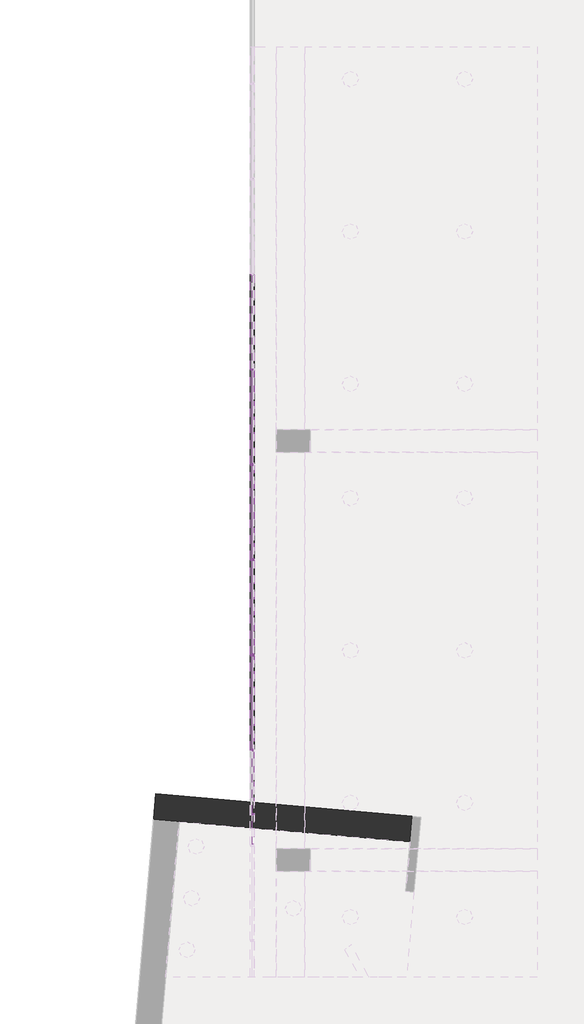
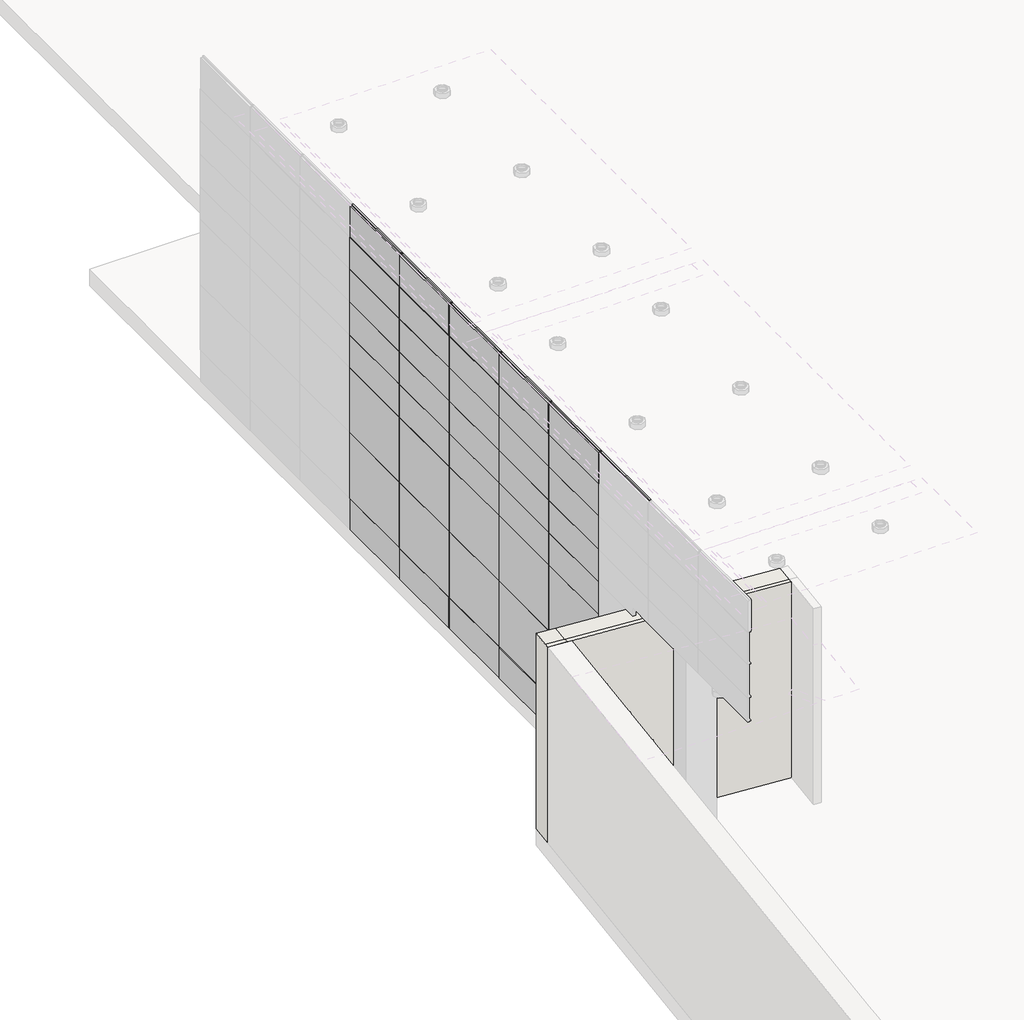
# One storey, part 6 of 30: 90 members, 40 plates, 1 wall.
# Revit data of these elements (continued)
# Space at (-48636.12, -949.776) mm, phase "New Construction", upper level "1ST. FL.", upper offset 3048 mm, lower offset 0 mm (continued)
#   Return Airflow = 0
#   Occupancy Unit = -1
#   Condition Type = 2
#   Construction Type = none
# Space at (-24605.823, -26109.518) mm, phase "New Construction", upper level "1ST. FL.", upper offset 3048 mm, lower offset 0 mm
#   Number = "165"
#   Name = "Space"
#   Actual Lighting Load per area = 0
#   Actual Power Load per area = 0
#   Sensible Heat Gain per person = 0
#   Specified Lighting Load = 11573.5 (stored number, unit not read)
#   Specified Power Load = 15045.5 (stored number, unit not read)
#   Latent Heat Gain per person = 0
#   Total Heat Gain per person = 0
#   Area per Person = 0
#   Number of People = 3.49616 (stored number, unit not read)
#   Lighting Load Units = 0
#   Power Load Units = 0
#   Return Airflow = 0
#   Occupancy Unit = -1
#   Condition Type = 2
#   Construction Type = none
# Space at (-26178.864, -19923.037) mm, phase "New Construction", upper level "1ST. FL.", upper offset 3048 mm, lower offset 0 mm
#   Number = "166"
#   Name = "Space"
#   Actual Lighting Load per area = 0
#   Actual Power Load per area = 0
#   Sensible Heat Gain per person = 0
#   Specified Lighting Load = 6526.22 (stored number, unit not read)
#   Specified Power Load = 8484.08 (stored number, unit not read)
#   Latent Heat Gain per person = 0
#   Total Heat Gain per person = 0
#   Area per Person = 0
#   Number of People = 1.97147 (stored number, unit not read)
#   Lighting Load Units = 0
#   Power Load Units = 0
#   Return Airflow = 0
#   Occupancy Unit = -1
#   Condition Type = 2
#   Construction Type = none
# Space at (-31002.156, -29519.268) mm, phase "New Construction", upper level "1ST. FL.", upper offset 3048 mm, lower offset 0 mm
#   Number = "167"
#   Name = "Space"
#   Actual Lighting Load per area = 0
#   Actual Power Load per area = 0
#   Sensible Heat Gain per person = 0
#   Specified Lighting Load = 1751.97 (stored number, unit not read)
#   Specified Power Load = 2277.57 (stored number, unit not read)
#   Latent Heat Gain per person = 0
#   Total Heat Gain per person = 0
#   Area per Person = 0
#   Number of People = 0.529244 (stored number, unit not read)
#   Lighting Load Units = 0
#   Power Load Units = 0
#   Return Airflow = 0
#   Occupancy Unit = -1
#   Condition Type = 2
#   Construction Type = none
# Space at (-35232.658, -22961.72) mm, phase "New Construction", upper level "1ST. FL.", upper offset 3048 mm, lower offset 0 mm
#   Number = "168"
#   Name = "Space"
#   Actual Lighting Load per area = 0
#   Actual Power Load per area = 0
#   Sensible Heat Gain per person = 0
#   Specified Lighting Load = 14661.4 (stored number, unit not read)
#   Specified Power Load = 19059.8 (stored number, unit not read)
#   Latent Heat Gain per person = 0
#   Total Heat Gain per person = 0
#   Area per Person = 0
#   Number of People = 4.42898 (stored number, unit not read)
#   Lighting Load Units = 0
#   Power Load Units = 0
#   Return Airflow = 0
#   Occupancy Unit = -1
#   Condition Type = 2
#   Construction Type = none
# Space at (-44559.948, -27773.147) mm, phase "New Construction", upper level "1ST. FL.", upper offset 3048 mm, lower offset 0 mm
#   Number = "6"
#   Name = "Space"
#   Actual Lighting Load per area = 0
#   Actual Power Load per area = 0
#   Sensible Heat Gain per person = 0
#   Specified Lighting Load = 153.554 (stored number, unit not read)
#   Specified Power Load = 199.62 (stored number, unit not read)
#   Latent Heat Gain per person = 0
#   Total Heat Gain per person = 0
#   Area per Person = 0
#   Number of People = 0.0463862 (stored number, unit not read)
#   Lighting Load Units = 0
#   Power Load Units = 0
#   Return Airflow = 0
#   Occupancy Unit = -1
#   Condition Type = 2
#   Construction Type = none
# Space at (-44641.303, -28703.045) mm, phase "New Construction", upper level "1ST. FL.", upper offset 3048 mm, lower offset 0 mm
#   Number = "7"
#   Name = "Space"
#   Actual Lighting Load per area = 0
#   Actual Power Load per area = 0
#   Sensible Heat Gain per person = 0
#   Specified Lighting Load = 153.554 (stored number, unit not read)
#   Specified Power Load = 199.62 (stored number, unit not read)
#   Latent Heat Gain per person = 0
#   Total Heat Gain per person = 0
#   Area per Person = 0
#   Number of People = 0.0463862 (stored number, unit not read)
#   Lighting Load Units = 0
#   Power Load Units = 0
#   Return Airflow = 0
#   Occupancy Unit = -1
#   Condition Type = 2
#   Construction Type = none
# Space at (-44722.659, -29632.943) mm, phase "New Construction", upper level "1ST. FL.", upper offset 3048 mm, lower offset 0 mm
#   Number = "8"
#   Name = "Space"
#   Actual Lighting Load per area = 0
#   Actual Power Load per area = 0
#   Sensible Heat Gain per person = 0
#   Specified Lighting Load = 153.554 (stored number, unit not read)
#   Specified Power Load = 199.62 (stored number, unit not read)
#   Latent Heat Gain per person = 0
#   Total Heat Gain per person = 0
#   Area per Person = 0
#   Number of People = 0.0463862 (stored number, unit not read)
#   Lighting Load Units = 0
#   Power Load Units = 0
#   Return Airflow = 0
#   Occupancy Unit = -1
#   Condition Type = 2
#   Construction Type = none
# Space at (4481.556, -17544.26) mm, phase "New Construction", upper level "1ST. FL.", upper offset 3048 mm, lower offset 0 mm
#   Number = "26"
#   Name = "Space"
#   Actual Lighting Load per area = 0
#   Actual Power Load per area = 0
#   Sensible Heat Gain per person = 0
#   Specified Lighting Load = 668.56 (stored number, unit not read)
#   Specified Power Load = 869.128 (stored number, unit not read)
#   Latent Heat Gain per person = 0
#   Total Heat Gain per person = 0
#   Area per Person = 0
#   Number of People = 0.201961 (stored number, unit not read)
#   Lighting Load Units = 0
#   Power Load Units = 0
#   Return Airflow = 0
#   Occupancy Unit = -1
#   Condition Type = 2
#   Construction Type = none
# Space at (13610.668, -16864.797) mm, phase "New Construction", upper level "1ST. FL.", upper offset 3048 mm, lower offset 0 mm
#   Number = "27"
#   Name = "Space"
#   Actual Lighting Load per area = 0
#   Actual Power Load per area = 0
#   Sensible Heat Gain per person = 0
#   Specified Lighting Load = 754.308 (stored number, unit not read)
#   Specified Power Load = 980.601 (stored number, unit not read)
#   Latent Heat Gain per person = 0
#   Total Heat Gain per person = 0
#   Area per Person = 0
#   Number of People = 0.227865 (stored number, unit not read)
#   Lighting Load Units = 0
#   Power Load Units = 0
#   Return Airflow = 0
#   Occupancy Unit = -1
#   Condition Type = 2
#   Construction Type = none
# Space at (16138.502, -11083.135) mm, phase "New Construction", upper level "1ST. FL.", upper offset 3048 mm, lower offset 0 mm
#   Number = "28"
#   Name = "Space"
#   Actual Lighting Load per area = 0
#   Actual Power Load per area = 0
#   Sensible Heat Gain per person = 0
#   Specified Lighting Load = 89.5362 (stored number, unit not read)
#   Specified Power Load = 116.397 (stored number, unit not read)
#   Latent Heat Gain per person = 0
#   Total Heat Gain per person = 0
#   Area per Person = 0
#   Number of People = 0.0270475 (stored number, unit not read)
#   Lighting Load Units = 0
#   Power Load Units = 0
#   Return Airflow = 0
#   Occupancy Unit = -1
#   Condition Type = 2
#   Construction Type = none
# Space at (-40541.142, -26152.586) mm, phase "New Construction", upper level "1ST. FL.", upper offset 3048 mm, lower offset 0 mm
#   Number = "3"
#   Name = "Space"
#   Actual Lighting Load per area = 0
#   Actual Power Load per area = 0
#   Sensible Heat Gain per person = 0
#   Specified Lighting Load = 4.78874 (stored number, unit not read)
#   Specified Power Load = 6.22536 (stored number, unit not read)
#   Latent Heat Gain per person = 0
#   Total Heat Gain per person = 0
#   Area per Person = 0
#   Number of People = 0.0014466 (stored number, unit not read)
#   Lighting Load Units = 0
#   Power Load Units = 0
#   Return Airflow = 0
#   Occupancy Unit = -1
#   Condition Type = 2
#   Construction Type = none
# Space at (-17133.844, -17937.396) mm, phase "New Construction", upper level "1ST. FL.", upper offset 3048 mm, lower offset 0 mm
#   Number = "32"
#   Name = "Space"
#   Actual Lighting Load per area = 0
#   Actual Power Load per area = 0
#   Sensible Heat Gain per person = 0
#   Specified Lighting Load = 933.723 (stored number, unit not read)
#   Specified Power Load = 1213.84 (stored number, unit not read)
#   Latent Heat Gain per person = 0
#   Total Heat Gain per person = 0
#   Area per Person = 0
#   Number of People = 0.282063 (stored number, unit not read)
#   Lighting Load Units = 0
#   Power Load Units = 0
#   Return Airflow = 0
#   Occupancy Unit = -1
#   Condition Type = 2
#   Construction Type = none
# Space at (-14581.144, -19075.025) mm, phase "New Construction", upper level "1ST. FL.", upper offset 3048 mm, lower offset 0 mm
#   Number = "33"
#   Name = "Space"
#   Actual Lighting Load per area = 0
#   Actual Power Load per area = 0
#   Sensible Heat Gain per person = 0
#   Specified Lighting Load = 79.3036 (stored number, unit not read)
#   Specified Power Load = 103.095 (stored number, unit not read)
#   Latent Heat Gain per person = 0
#   Total Heat Gain per person = 0
#   Area per Person = 0
#   Number of People = 0.0239564 (stored number, unit not read)
#   Lighting Load Units = 0
#   Power Load Units = 0
#   Return Airflow = 0
#   Occupancy Unit = -1
#   Condition Type = 2
#   Construction Type = none
# Space at (-36860.119, -18528.984) mm, phase "New Construction", upper level "1ST. FL.", upper offset 3048 mm, lower offset 0 mm
#   Number = "34"
#   Name = "Space"
#   Actual Lighting Load per area = 0
#   Actual Power Load per area = 0
#   Sensible Heat Gain per person = 0
#   Specified Lighting Load = 2950.45 (stored number, unit not read)
#   Specified Power Load = 3835.59 (stored number, unit not read)
#   Latent Heat Gain per person = 0
#   Total Heat Gain per person = 0
#   Area per Person = 0
#   Number of People = 0.891285 (stored number, unit not read)
#   Lighting Load Units = 0
#   Power Load Units = 0
#   Return Airflow = 0
#   Occupancy Unit = -1
#   Condition Type = 2
#   Construction Type = none
# Space at (15225.756, 13850.14) mm, phase "New Construction", upper level "1ST. FL.", upper offset 3048 mm, lower offset 0 mm
#   Number = "35"
#   Name = "Space"
#   Actual Lighting Load per area = 0
#   Actual Power Load per area = 0
#   Sensible Heat Gain per person = 0
#   Specified Lighting Load = 62.8642 (stored number, unit not read)
#   Specified Power Load = 81.7235 (stored number, unit not read)
#   Latent Heat Gain per person = 0
#   Total Heat Gain per person = 0
#   Area per Person = 0
#   Number of People = 0.0189903 (stored number, unit not read)
#   Lighting Load Units = 0
#   Power Load Units = 0
#   Return Airflow = 0
#   Occupancy Unit = -1
#   Condition Type = 2
#   Construction Type = none
# Space at (-44280.616, -26218.59) mm, phase "New Construction", upper level "1ST. FL.", upper offset 3048 mm, lower offset 0 mm
#   Number = "4"
#   Name = "Space"
#   Actual Lighting Load per area = 0
#   Actual Power Load per area = 0
#   Sensible Heat Gain per person = 0
#   Specified Lighting Load = 35.218 (stored number, unit not read)
#   Specified Power Load = 45.7834 (stored number, unit not read)
#   Latent Heat Gain per person = 0
#   Total Heat Gain per person = 0
#   Area per Person = 0
#   Number of People = 0.0106388 (stored number, unit not read)
#   Lighting Load Units = 0
#   Power Load Units = 0
#   Return Airflow = 0
#   Occupancy Unit = -1
#   Condition Type = 2
#   Construction Type = none
# Space at (-44388.044, 13850.14) mm, phase "New Construction", upper level "1ST. FL.", upper offset 3048 mm, lower offset 0 mm
#   Number = "38"
#   Name = "Space"
#   Actual Lighting Load per area = 0
#   Actual Power Load per area = 0
#   Sensible Heat Gain per person = 0
#   Specified Lighting Load = 62.8642 (stored number, unit not read)
#   Specified Power Load = 81.7235 (stored number, unit not read)
#   Latent Heat Gain per person = 0
#   Total Heat Gain per person = 0
#   Area per Person = 0
#   Number of People = 0.0189903 (stored number, unit not read)
#   Lighting Load Units = 0
#   Power Load Units = 0
#   Return Airflow = 0
#   Occupancy Unit = -1
#   Condition Type = 2
#   Construction Type = none
# Space at (-49662.767, -15921.188) mm, phase "New Construction", upper level "1ST. FL.", upper offset 3048 mm, lower offset 0 mm
#   Number = "1"
#   Name = "Space"
#   Actual Lighting Load per area = 0
#   Actual Power Load per area = 0
#   Sensible Heat Gain per person = 0
#   Specified Lighting Load = 10.6063 (stored number, unit not read)
#   Specified Power Load = 13.7882 (stored number, unit not read)
#   Latent Heat Gain per person = 0
#   Total Heat Gain per person = 0
#   Area per Person = 0
#   Number of People = 0.003204 (stored number, unit not read)
#   Lighting Load Units = 0
#   Power Load Units = 0
#   Return Airflow = 0
#   Occupancy Unit = -1
#   Condition Type = 2
#   Construction Type = none
# Space at (-14581.144, 13850.14) mm, phase "New Construction", upper level "1ST. FL.", upper offset 3048 mm, lower offset 0 mm
#   Number = "39"
#   Name = "Space"
#   Actual Lighting Load per area = 0
#   Actual Power Load per area = 0
#   Sensible Heat Gain per person = 0
#   Specified Lighting Load = 134.399 (stored number, unit not read)
#   Specified Power Load = 174.719 (stored number, unit not read)
#   Latent Heat Gain per person = 0
#   Total Heat Gain per person = 0
#   Area per Person = 0
#   Number of People = 0.0405999 (stored number, unit not read)
#   Lighting Load Units = 0
#   Power Load Units = 0
#   Return Airflow = 0
#   Occupancy Unit = -1
#   Condition Type = 2
#   Construction Type = none
# Space at (-27319.244, 18968.24) mm, phase "New Construction", upper level "1ST. FL.", upper offset 3048 mm, lower offset 0 mm
#   Number = "42"
#   Name = "Space"
#   Actual Lighting Load per area = 0
#   Actual Power Load per area = 0
#   Sensible Heat Gain per person = 0
#   Specified Lighting Load = 63.238 (stored number, unit not read)
#   Specified Power Load = 82.2094 (stored number, unit not read)
#   Latent Heat Gain per person = 0
#   Total Heat Gain per person = 0
#   Area per Person = 0
#   Number of People = 0.0191032 (stored number, unit not read)
#   Lighting Load Units = 0
#   Power Load Units = 0
#   Return Airflow = 0
#   Occupancy Unit = -1
#   Condition Type = 2
#   Construction Type = none
# Space at (-26039.719, 18968.24) mm, phase "New Construction", upper level "1ST. FL.", upper offset 3048 mm, lower offset 0 mm
#   Number = "43"
#   Name = "Space"
#   Actual Lighting Load per area = 0
#   Actual Power Load per area = 0
#   Sensible Heat Gain per person = 0
#   Specified Lighting Load = 552.454 (stored number, unit not read)
#   Specified Power Load = 718.19 (stored number, unit not read)
#   Latent Heat Gain per person = 0
#   Total Heat Gain per person = 0
#   Area per Person = 0
#   Number of People = 0.166888 (stored number, unit not read)
#   Lighting Load Units = 0
#   Power Load Units = 0
#   Return Airflow = 0
#   Occupancy Unit = -1
#   Condition Type = 2
#   Construction Type = none
# Space at (15806.781, -12603.96) mm, phase "New Construction", upper level "1ST. FL.", upper offset 3048 mm, lower offset 0 mm
#   Number = "60"
#   Name = "Space"
#   Actual Lighting Load per area = 0
#   Actual Power Load per area = 0
#   Sensible Heat Gain per person = 0
#   Specified Lighting Load = 3.50388 (stored number, unit not read)
#   Specified Power Load = 4.55504 (stored number, unit not read)
#   Latent Heat Gain per person = 0
#   Total Heat Gain per person = 0
#   Area per Person = 0
#   Number of People = 0.00105847 (stored number, unit not read)
#   Lighting Load Units = 0
#   Power Load Units = 0
#   Return Airflow = 0
#   Occupancy Unit = -1
#   Condition Type = 2
#   Construction Type = none
# Space at (-44850.987, -31099.746) mm, phase "New Construction", upper level "1ST. FL.", upper offset 3048 mm, lower offset 0 mm
#   Number = "9"
#   Name = "Space"
#   Actual Lighting Load per area = 0
#   Actual Power Load per area = 0
#   Sensible Heat Gain per person = 0
#   Specified Lighting Load = 352.476 (stored number, unit not read)
#   Specified Power Load = 458.219 (stored number, unit not read)
#   Latent Heat Gain per person = 0
#   Total Heat Gain per person = 0
#   Area per Person = 0
#   Number of People = 0.106477 (stored number, unit not read)
#   Lighting Load Units = 0
#   Power Load Units = 0
#   Return Airflow = 0
#   Occupancy Unit = -1
#   Condition Type = 2
#   Construction Type = none
# Space at (15806.781, -5898.36) mm, phase "New Construction", upper level "1ST. FL.", upper offset 3048 mm, lower offset 0 mm
#   Number = "61"
#   Name = "Space"
#   Actual Lighting Load per area = 0
#   Actual Power Load per area = 0
#   Sensible Heat Gain per person = 0
#   Specified Lighting Load = 3.50388 (stored number, unit not read)
#   Specified Power Load = 4.55504 (stored number, unit not read)
#   Latent Heat Gain per person = 0
#   Total Heat Gain per person = 0
#   Area per Person = 0
#   Number of People = 0.00105847 (stored number, unit not read)
#   Lighting Load Units = 0
#   Power Load Units = 0
#   Return Airflow = 0
#   Occupancy Unit = -1
#   Condition Type = 2
#   Construction Type = none
# Space at (-41141.59, -31068.115) mm, phase "New Construction", upper level "1ST. FL.", upper offset 3048 mm, lower offset 0 mm
#   Number = "2"
#   Name = "Space"
#   Actual Lighting Load per area = 0
#   Actual Power Load per area = 0
#   Sensible Heat Gain per person = 0
#   Specified Lighting Load = 101.303 (stored number, unit not read)
#   Specified Power Load = 131.694 (stored number, unit not read)
#   Latent Heat Gain per person = 0
#   Total Heat Gain per person = 0
#   Area per Person = 0
#   Number of People = 0.030602 (stored number, unit not read)
#   Lighting Load Units = 0
#   Power Load Units = 0
#   Return Airflow = 0
#   Occupancy Unit = -1
#   Condition Type = 2
#   Construction Type = none
# Space at (-46265.71, -27605.083) mm, phase "New Construction", upper level "1ST. FL.", upper offset 3048 mm, lower offset 0 mm
#   Number = "10"
#   Name = "Space"
#   Actual Lighting Load per area = 0
#   Actual Power Load per area = 0
#   Sensible Heat Gain per person = 0
#   Specified Lighting Load = 198.964 (stored number, unit not read)
#   Specified Power Load = 258.653 (stored number, unit not read)
#   Latent Heat Gain per person = 0
#   Total Heat Gain per person = 0
#   Area per Person = 0
#   Number of People = 0.0601039 (stored number, unit not read)
#   Lighting Load Units = 0
#   Power Load Units = 0
#   Return Airflow = 0
#   Occupancy Unit = -1
#   Condition Type = 2
#   Construction Type = none
# Space at (-47287.648, -27585.498) mm, phase "New Construction", upper level "1ST. FL.", upper offset 3048 mm, lower offset 0 mm
#   Number = "11"
#   Name = "Space"
#   Actual Lighting Load per area = 0
#   Actual Power Load per area = 0
#   Sensible Heat Gain per person = 0
#   Specified Lighting Load = 153.554 (stored number, unit not read)
#   Specified Power Load = 199.62 (stored number, unit not read)
#   Latent Heat Gain per person = 0
#   Total Heat Gain per person = 0
#   Area per Person = 0
#   Number of People = 0.0463862 (stored number, unit not read)
#   Lighting Load Units = 0
#   Power Load Units = 0
#   Return Airflow = 0
#   Occupancy Unit = -1
#   Condition Type = 2
#   Construction Type = none
# Space at (-50077.342, -27341.431) mm, phase "New Construction", upper level "1ST. FL.", upper offset 3048 mm, lower offset 0 mm
#   Number = "14"
#   Name = "Space"
#   Actual Lighting Load per area = 0
#   Actual Power Load per area = 0
#   Sensible Heat Gain per person = 0
#   Specified Lighting Load = 153.554 (stored number, unit not read)
#   Specified Power Load = 199.62 (stored number, unit not read)
#   Latent Heat Gain per person = 0
#   Total Heat Gain per person = 0
#   Area per Person = 0
#   Number of People = 0.0463862 (stored number, unit not read)
#   Lighting Load Units = 0
#   Power Load Units = 0
#   Return Airflow = 0
#   Occupancy Unit = -1
#   Condition Type = 2
#   Construction Type = none
# Space at (29814.881, 10827.54) mm, phase "New Construction", upper level "1ST. FL.", upper offset 3048 mm, lower offset 0 mm
#   Number = "86"
#   Name = "Space"
#   Actual Lighting Load per area = 0
#   Actual Power Load per area = 0
#   Sensible Heat Gain per person = 0
#   Specified Lighting Load = 153.554 (stored number, unit not read)
#   Specified Power Load = 199.62 (stored number, unit not read)
#   Latent Heat Gain per person = 0
#   Total Heat Gain per person = 0
#   Area per Person = 0
#   Number of People = 0.0463862 (stored number, unit not read)
#   Lighting Load Units = 0
#   Power Load Units = 0
#   Return Airflow = 0
#   Occupancy Unit = -1
#   Condition Type = 2
#   Construction Type = none
# Space at (-51007.239, -27260.076) mm, phase "New Construction", upper level "1ST. FL.", upper offset 3048 mm, lower offset 0 mm
#   Number = "15"
#   Name = "Space"
#   Actual Lighting Load per area = 0
#   Actual Power Load per area = 0
#   Sensible Heat Gain per person = 0
#   Specified Lighting Load = 153.554 (stored number, unit not read)
#   Specified Power Load = 199.62 (stored number, unit not read)
#   Latent Heat Gain per person = 0
#   Total Heat Gain per person = 0
#   Area per Person = 0
#   Number of People = 0.0463862 (stored number, unit not read)
#   Lighting Load Units = 0
#   Power Load Units = 0
#   Return Airflow = 0
#   Occupancy Unit = -1
#   Condition Type = 2
#   Construction Type = none
# Space at (-47010.699, -30758.61) mm, phase "New Construction", upper level "1ST. FL.", upper offset 3048 mm, lower offset 0 mm
#   Number = "17"
#   Name = "Space"
#   Actual Lighting Load per area = 0
#   Actual Power Load per area = 0
#   Sensible Heat Gain per person = 0
#   Specified Lighting Load = 352.476 (stored number, unit not read)
#   Specified Power Load = 458.219 (stored number, unit not read)
#   Latent Heat Gain per person = 0
#   Total Heat Gain per person = 0
#   Area per Person = 0
#   Number of People = 0.106477 (stored number, unit not read)
#   Lighting Load Units = 0
#   Power Load Units = 0
#   Return Airflow = 0
#   Occupancy Unit = -1
#   Condition Type = 2
#   Construction Type = none
# Space at (28636.162, 6964.942) mm, phase "New Construction", upper level "1ST. FL.", upper offset 3048 mm, lower offset 0 mm
#   Number = "101"
#   Name = "Space"
#   Actual Lighting Load per area = 0
#   Actual Power Load per area = 0
#   Sensible Heat Gain per person = 0
#   Specified Lighting Load = 2584.91 (stored number, unit not read)
#   Specified Power Load = 3360.39 (stored number, unit not read)
#   Latent Heat Gain per person = 0
#   Total Heat Gain per person = 0
#   Area per Person = 0
#   Number of People = 0.780861 (stored number, unit not read)
#   Lighting Load Units = 0
#   Power Load Units = 0
#   Return Airflow = 0
#   Occupancy Unit = -1
#   Condition Type = 2
#   Construction Type = none
# Space at (-25325.344, 24245.09) mm, phase "New Construction", upper level "1ST. FL.", upper offset 3048 mm, lower offset 0 mm
#   Number = "52"
#   Name = "Space"
#   Actual Lighting Load per area = 0
#   Actual Power Load per area = 0
#   Sensible Heat Gain per person = 0
#   Specified Lighting Load = 1393.93 (stored number, unit not read)
#   Specified Power Load = 1812.1 (stored number, unit not read)
#   Latent Heat Gain per person = 0
#   Total Heat Gain per person = 0
#   Area per Person = 0
#   Number of People = 0.421083 (stored number, unit not read)
#   Lighting Load Units = 0
#   Power Load Units = 0
#   Return Airflow = 0
#   Occupancy Unit = -1
#   Condition Type = 2
#   Construction Type = none
# Space at (-48217.546, -27504.142) mm, phase "New Construction", upper level "1ST. FL.", upper offset 3048 mm, lower offset 0 mm
#   Number = "12"
#   Name = "Space"
#   Actual Lighting Load per area = 0
#   Actual Power Load per area = 0
#   Sensible Heat Gain per person = 0
#   Specified Lighting Load = 153.554 (stored number, unit not read)
#   Specified Power Load = 199.62 (stored number, unit not read)
#   Latent Heat Gain per person = 0
#   Total Heat Gain per person = 0
#   Area per Person = 0
#   Number of People = 0.0463862 (stored number, unit not read)
#   Lighting Load Units = 0
#   Power Load Units = 0
#   Return Airflow = 0
#   Occupancy Unit = -1
#   Condition Type = 2
#   Construction Type = none
# Space at (-49147.444, -27422.787) mm, phase "New Construction", upper level "1ST. FL.", upper offset 3048 mm, lower offset 0 mm
#   Number = "13"
#   Name = "Space"
#   Actual Lighting Load per area = 0
#   Actual Power Load per area = 0
#   Sensible Heat Gain per person = 0
#   Specified Lighting Load = 153.554 (stored number, unit not read)
#   Specified Power Load = 199.62 (stored number, unit not read)
#   Latent Heat Gain per person = 0
#   Total Heat Gain per person = 0
#   Area per Person = 0
#   Number of People = 0.0463862 (stored number, unit not read)
#   Lighting Load Units = 0
#   Power Load Units = 0
#   Return Airflow = 0
#   Occupancy Unit = -1
#   Condition Type = 2
#   Construction Type = none
# Space at (-51937.137, -27178.72) mm, phase "New Construction", upper level "1ST. FL.", upper offset 3048 mm, lower offset 0 mm
#   Number = "16"
#   Name = "Space"
#   Actual Lighting Load per area = 0
#   Actual Power Load per area = 0
#   Sensible Heat Gain per person = 0
#   Specified Lighting Load = 153.554 (stored number, unit not read)
#   Specified Power Load = 199.62 (stored number, unit not read)
#   Latent Heat Gain per person = 0
#   Total Heat Gain per person = 0
#   Area per Person = 0
#   Number of People = 0.0463862 (stored number, unit not read)
#   Lighting Load Units = 0
#   Power Load Units = 0
#   Return Airflow = 0
#   Occupancy Unit = -1
#   Condition Type = 2
#   Construction Type = none
# Space at (-48490.944, -30629.106) mm, phase "New Construction", upper level "1ST. FL.", upper offset 3048 mm, lower offset 0 mm
#   Number = "18"
#   Name = "Space"
#   Actual Lighting Load per area = 0
#   Actual Power Load per area = 0
#   Sensible Heat Gain per person = 0
#   Specified Lighting Load = 153.554 (stored number, unit not read)
#   Specified Power Load = 199.62 (stored number, unit not read)
#   Latent Heat Gain per person = 0
#   Total Heat Gain per person = 0
#   Area per Person = 0
#   Number of People = 0.0463862 (stored number, unit not read)
#   Lighting Load Units = 0
#   Power Load Units = 0
#   Return Airflow = 0
#   Occupancy Unit = -1
#   Condition Type = 2
#   Construction Type = none
# Space at (-49420.842, -30547.75) mm, phase "New Construction", upper level "1ST. FL.", upper offset 3048 mm, lower offset 0 mm
#   Number = "19"
#   Name = "Space"
#   Actual Lighting Load per area = 0
#   Actual Power Load per area = 0
#   Sensible Heat Gain per person = 0
#   Specified Lighting Load = 153.554 (stored number, unit not read)
#   Specified Power Load = 199.62 (stored number, unit not read)
#   Latent Heat Gain per person = 0
#   Total Heat Gain per person = 0
#   Area per Person = 0
#   Number of People = 0.0463862 (stored number, unit not read)
#   Lighting Load Units = 0
#   Power Load Units = 0
#   Return Airflow = 0
#   Occupancy Unit = -1
#   Condition Type = 2
#   Construction Type = none
# Space at (-8153.499, -33698.818) mm, phase "New Construction", upper level "1ST. FL.", upper offset 3048 mm, lower offset 0 mm
#   Number = "113"
#   Name = "Space"
#   Actual Lighting Load per area = 0
#   Actual Power Load per area = 0
#   Sensible Heat Gain per person = 0
#   Specified Lighting Load = 1924.29 (stored number, unit not read)
#   Specified Power Load = 2501.58 (stored number, unit not read)
#   Latent Heat Gain per person = 0
#   Total Heat Gain per person = 0
#   Area per Person = 0
#   Number of People = 0.581298 (stored number, unit not read)
#   Lighting Load Units = 0
#   Power Load Units = 0
#   Return Airflow = 0
#   Occupancy Unit = -1
#   Condition Type = 2
#   Construction Type = none
# Space at (11055.612, -25627.612) mm, phase "New Construction", upper level "1ST. FL.", upper offset 3048 mm, lower offset 0 mm
#   Number = "118"
#   Name = "Space"
#   Actual Lighting Load per area = 0
#   Actual Power Load per area = 0
#   Sensible Heat Gain per person = 0
#   Specified Lighting Load = 2533.2 (stored number, unit not read)
#   Specified Power Load = 3293.16 (stored number, unit not read)
#   Latent Heat Gain per person = 0
#   Total Heat Gain per person = 0
#   Area per Person = 0
#   Number of People = 0.765241 (stored number, unit not read)
#   Lighting Load Units = 0
#   Power Load Units = 0
#   Return Airflow = 0
#   Occupancy Unit = -1
#   Condition Type = 2
#   Construction Type = none
# Space at (-42695.927, -18100.252) mm, phase "New Construction", upper level "1ST. FL.", upper offset 3048 mm, lower offset 0 mm
#   Number = "25"
#   Name = "Space"
#   Actual Lighting Load per area = 0
#   Actual Power Load per area = 0
#   Sensible Heat Gain per person = 0
#   Specified Lighting Load = 774.034 (stored number, unit not read)
#   Specified Power Load = 1006.24 (stored number, unit not read)
#   Latent Heat Gain per person = 0
#   Total Heat Gain per person = 0
#   Area per Person = 0
#   Number of People = 0.233824 (stored number, unit not read)
#   Lighting Load Units = 0
#   Power Load Units = 0
#   Return Airflow = 0
#   Occupancy Unit = -1
#   Condition Type = 2
#   Construction Type = none
# Space at (-44477.762, -26833.76) mm, phase "New Construction", upper level "1ST. FL.", upper offset 3048 mm, lower offset 0 mm
#   Number = "5"
#   Name = "Space"
#   Actual Lighting Load per area = 0
#   Actual Power Load per area = 0
#   Sensible Heat Gain per person = 0
#   Specified Lighting Load = 153.554 (stored number, unit not read)
#   Specified Power Load = 199.62 (stored number, unit not read)
#   Latent Heat Gain per person = 0
#   Total Heat Gain per person = 0
#   Area per Person = 0
#   Number of People = 0.0463862 (stored number, unit not read)
#   Lighting Load Units = 0
#   Power Load Units = 0
#   Return Airflow = 0
#   Occupancy Unit = -1
#   Condition Type = 2
#   Construction Type = none
# Space at (19016.617, -16733.72) mm, phase "New Construction", upper level "1ST. FL.", upper offset 3048 mm, lower offset 0 mm
#   Number = "164"
#   Name = "Space"
#   Actual Lighting Load per area = 0
#   Actual Power Load per area = 0
#   Sensible Heat Gain per person = 0
#   Specified Lighting Load = 47834 (stored number, unit not read)
#   Specified Power Load = 62184.2 (stored number, unit not read)
#   Latent Heat Gain per person = 0
#   Total Heat Gain per person = 0
#   Area per Person = 0
#   Number of People = 14.4499 (stored number, unit not read)
#   Lighting Load Units = 0
#   Power Load Units = 0
#   Return Airflow = 0
#   Occupancy Unit = -1
#   Condition Type = 2
#   Construction Type = none
# Space at (9936.299, -25451.788) mm, phase "New Construction", upper level "1ST. FL.", upper offset 3048 mm, lower offset 0 mm
#   Number = "116"
#   Name = "Space"
#   Actual Lighting Load per area = 0
#   Actual Power Load per area = 0
#   Sensible Heat Gain per person = 0
#   Specified Lighting Load = 37.5245 (stored number, unit not read)
#   Specified Power Load = 48.7818 (stored number, unit not read)
#   Latent Heat Gain per person = 0
#   Total Heat Gain per person = 0
#   Area per Person = 0
#   Number of People = 0.0113355 (stored number, unit not read)
#   Lighting Load Units = 0
#   Power Load Units = 0
#   Return Airflow = 0
#   Occupancy Unit = -1
#   Condition Type = 2
#   Construction Type = none
